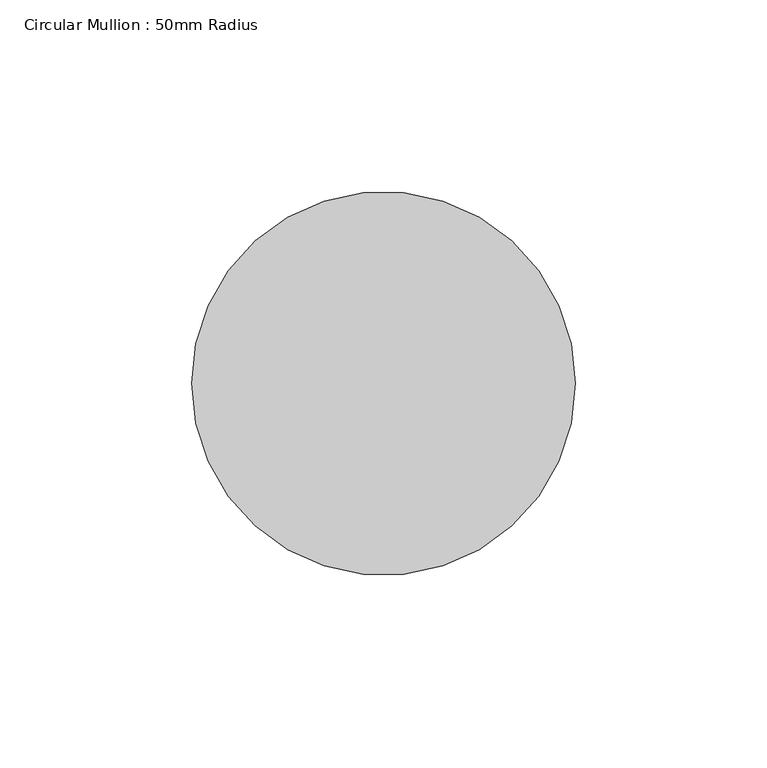
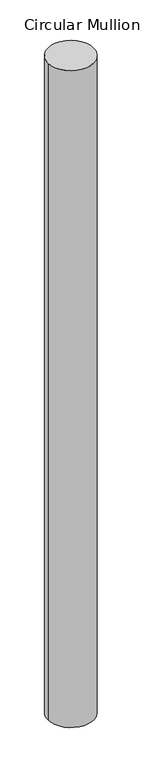
"""IFC4 building model written with IfcOpenShell, lengths in millimetres: member geometry, Circular Mullion : 50mm Radius."""

from ifc_helpers import new_model, si_unit, point, frame, origin, origin_2d, place, context, project, spatial, circle_curve, trimmed, segment, composite_curve, outline, extrude, source, transform, mapped, element, save


def circular_mullion_50mm_radius_4f14ee8a(model_context):
    return source(origin(), model_context, "Body", "SweptSolid", [
        extrude(outline(composite_curve([segment(trimmed(circle_curve(origin_2d(), 50.0), [point((50.0, 0.0))], [point((-50.0, 0.0))], False, "CARTESIAN"), True, "CONTINUOUS"), segment(trimmed(circle_curve(origin_2d(), 50.0), [point((-50.0, 0.0))], [point((50.0, 0.0))], False, "CARTESIAN"), True, "CONTINUOUS")], self_intersect=False)), frame((0.0, 0.0, -1516.7668663), z_axis=(0.0, 0.0, 1.0), x_axis=(1.0, 0.0, 0.0)), (0.0, 0.0, 1.0), 1516.7668663),
    ])


if __name__ == "__main__":
    model = new_model("IFC4")
    model_context = context("Model", 3, world=origin())
    ifc_project = project(units=[si_unit("LENGTHUNIT", "METRE", prefix="MILLI")], contexts=[model_context])
    site = spatial("IfcSite", under=ifc_project)
    building = spatial("IfcBuilding", under=site)
    placement = place(None, origin())
    circular_mullion_50mm_radius_shape = circular_mullion_50mm_radius_4f14ee8a(model_context)
    element("IfcMember", 1, ObjectType="Circular Mullion : 50mm Radius", at=placement, inside=building, context=model_context, shape_type="MappedRepresentation", body=[
        mapped(circular_mullion_50mm_radius_shape, transform((0.0, 0.0, 0.0), x_axis=(1.0, 0.0, 0.0), y_axis=(0.0, 1.0, 0.0), z_axis=(0.0, 0.0, 1.0))),
    ])
    save(model, "model.ifc")

# Revit data of these elements
# Type "Circular Mullion : 50mm Radius"
#   built-in parameter 1007350 = 0.164042 (stored number, unit not read)
# Element 1 (IfcMember, "Circular Mullion : 50mm Radius")
#   Materials on its faces: "Aluminium"
# Materials
#   "Aluminium": class "Metal", colour RGB 247 247 247, transparency 0, Description = "Aluminium 6061", Cost = 0
